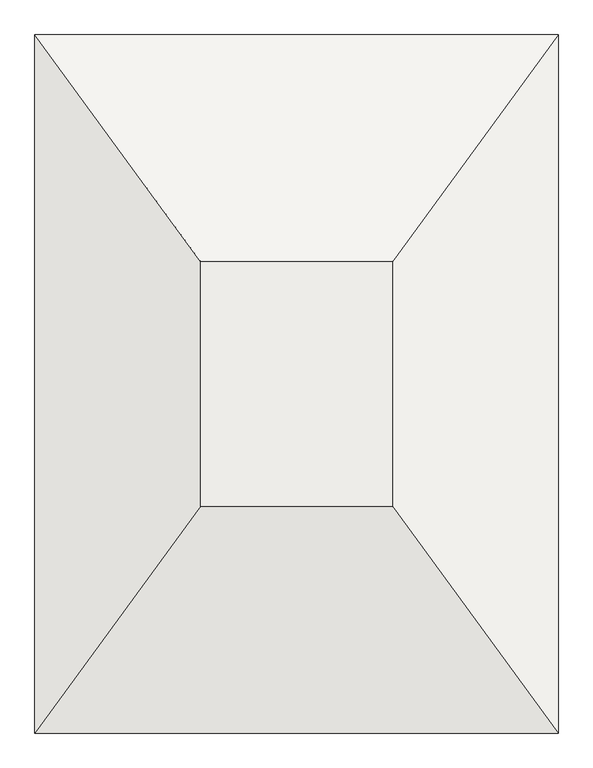
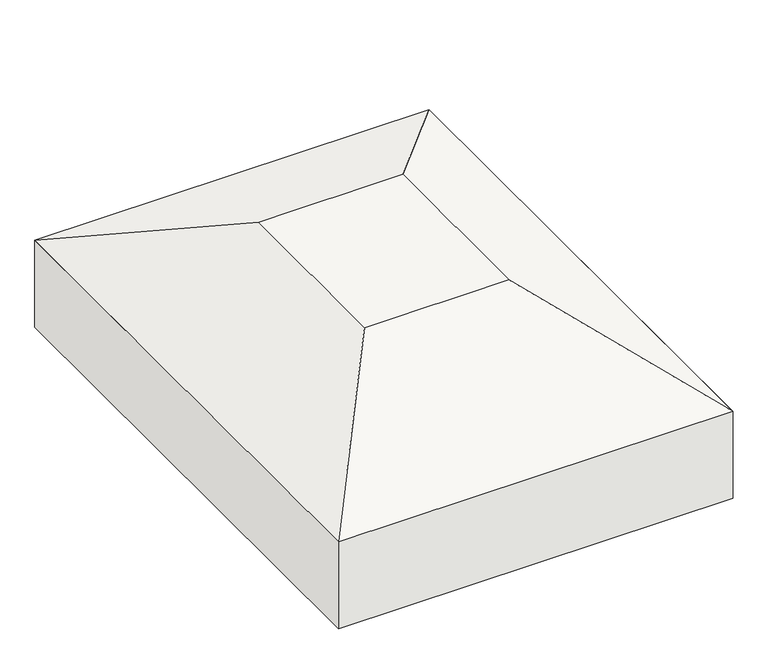
"""IFC4 building model written with IfcOpenShell, lengths in millimetres: slab geometry, 独立基础 - 坡形截面 : 独立基础 - 坡形截面."""

import ifcopenshell
import ifcopenshell.guid

model = None  # the IFC model being written
_history = None  # IfcOwnerHistory: only IFC2X3 demands one
_inside = {}  # id of a spatial element -> (the spatial element, [elements in it])
_under = {}  # id of a project, library or spatial element -> (it, [spatial elements below it])
_declared = {}  # id of a project -> (the project, [libraries it declares])
_typed = {}  # id of a type object -> (the type object, [elements of that type])
_made_of = {}  # id of a material, layer set ... -> (it, [elements and type objects made of it])


def new_model(schema):
    """Start an empty IFC model of exactly this schema.

    Asked for "IFC4X3", IfcOpenShell would pick the latest addendum, in which some entities
    have other attributes; the version numbers below select the first issue.
    IFC2X3 requires an IfcOwnerHistory on every rooted entity: one is made here for all.
    """
    global model, _history
    if schema == "IFC4X3":
        model = ifcopenshell.file(schema_version=(4, 3, 0, 0))
    else:
        model = ifcopenshell.file(schema=schema)
    _inside.clear()
    _under.clear()
    _declared.clear()
    _typed.clear()
    _made_of.clear()
    _history = None
    if model.schema == "IFC2X3":
        org = make("IfcOrganization", Name="unknown")
        user = make(
            "IfcPersonAndOrganization",
            ThePerson=make("IfcPerson", FamilyName="unknown"),
            TheOrganization=org,
        )
        app = make(
            "IfcApplication",
            ApplicationDeveloper=org,
            Version="unknown",
            ApplicationFullName="unknown",
            ApplicationIdentifier="unknown",
        )
        _history = make(
            "IfcOwnerHistory",
            OwningUser=user,
            OwningApplication=app,
            ChangeAction="ADDED",
            CreationDate=0,
        )
    return model


def make(cls, **values):
    """One entity of the class cls with the attributes given. An attribute that is None is left unset."""
    return model.create_entity(
        cls, **{name: value for name, value in values.items() if value is not None}
    )


def rooted(cls, **values):
    """An entity with a GlobalId (a new one), such as an element, a storey or a relation."""
    return make(cls, GlobalId=ifcopenshell.guid.new(), OwnerHistory=_history, **values)


def si_unit(unit_type, name, prefix=None):
    """IfcSIUnit, for example si_unit("LENGTHUNIT", "METRE", prefix="MILLI")."""
    return make("IfcSIUnit", UnitType=unit_type, Prefix=prefix, Name=name)


def assignment(units):
    """IfcUnitAssignment: the units of a project."""
    return None if units is None else make("IfcUnitAssignment", Units=units)


def point(xyz):
    """IfcCartesianPoint."""
    return None if xyz is None else make("IfcCartesianPoint", Coordinates=xyz)


def direction(xyz):
    """IfcDirection."""
    return None if xyz is None else make("IfcDirection", DirectionRatios=xyz)


def frame(location, z_axis=None, x_axis=None):
    """IfcAxis2Placement3D, a coordinate frame: its origin and axes. An axis left out is left unset."""
    return make(
        "IfcAxis2Placement3D",
        Location=point(location),
        Axis=direction(z_axis),
        RefDirection=direction(x_axis),
    )


def origin():
    """The frame at (0, 0, 0) with its axes left unset."""
    return frame((0.0, 0.0, 0.0))


def place(relative_to, where):
    """IfcLocalPlacement: puts the frame where relative to a parent placement (None: the world)."""
    return make(
        "IfcLocalPlacement", PlacementRelTo=relative_to, RelativePlacement=where
    )


def context(
    kind, dimensions, precision=None, world=None, true_north=None, identifier=None
):
    """IfcGeometricRepresentationContext, for example the 3D "Model" context."""
    return make(
        "IfcGeometricRepresentationContext",
        ContextIdentifier=identifier,
        ContextType=kind,
        CoordinateSpaceDimension=dimensions,
        Precision=precision,
        WorldCoordinateSystem=world,
        TrueNorth=true_north,
    )


def project(units=None, contexts=None):
    """IfcProject with its units and contexts."""
    return rooted(
        "IfcProject",
        Name="project",
        RepresentationContexts=contexts,
        UnitsInContext=assignment(units),
    )


def spatial(cls, under=None, at=None, **own):
    """A site, building, storey or space (cls), placed at a placement, below another one or the project."""
    s = rooted(cls, ObjectPlacement=at, **own)
    if under is not None:
        _under.setdefault(under.id(), (under, []))[1].append(s)
    return s


def polyline(points):
    """IfcPolyline through the points."""
    return make("IfcPolyline", Points=[point(p) for p in points])


def outline(outer, holes=None, kind="AREA"):
    """IfcArbitraryClosedProfileDef: a profile drawn as a closed curve; with holes, ...WithVoids."""
    if holes is None:
        return make("IfcArbitraryClosedProfileDef", ProfileType=kind, OuterCurve=outer)
    return make(
        "IfcArbitraryProfileDefWithVoids",
        ProfileType=kind,
        OuterCurve=outer,
        InnerCurves=holes,
    )


def extrude(swept, where, along, depth):
    """IfcExtrudedAreaSolid: the profile swept, set in the frame where, extruded along a direction by depth."""
    return make(
        "IfcExtrudedAreaSolid",
        SweptArea=swept,
        Position=where,
        ExtrudedDirection=direction(along),
        Depth=depth,
    )


def faces_of(points, faces, orient=None, outer=None):
    """IfcFace entities. A face is a list of loops; a loop is a list of indices into points, from 0.

    orient and outer hold one flag for each loop. By default every Orientation is true, the
    first loop of a face is its IfcFaceOuterBound and the others are IfcFaceBound.
    """
    made = []
    for i, loops in enumerate(faces):
        bounds = []
        for j, loop in enumerate(loops):
            is_outer = j == 0 if outer is None else outer[i][j]
            bounds.append(
                make(
                    "IfcFaceOuterBound" if is_outer else "IfcFaceBound",
                    Bound=make("IfcPolyLoop", Polygon=[points[k] for k in loop]),
                    Orientation=True if orient is None else orient[i][j],
                )
            )
        made.append(make("IfcFace", Bounds=bounds))
    return made


def faceted_brep(points, faces, orient=None, outer=None, voids=None):
    """IfcFacetedBrep: a solid bounded by flat faces; with voids (closed shells), ...WithVoids."""
    shared = [point(p) for p in points]
    hull = make("IfcClosedShell", CfsFaces=faces_of(shared, faces, orient, outer))
    if voids is None:
        return make("IfcFacetedBrep", Outer=hull)
    return make(
        "IfcFacetedBrepWithVoids",
        Outer=hull,
        Voids=[
            make(cls, CfsFaces=faces_of(shared, fs, o, b)) for cls, fs, o, b in voids
        ],
    )


def shape(context_of_items, identifier, shape_type, items):
    """IfcShapeRepresentation: the items that make up one representation, for example the "Body"."""
    return make(
        "IfcShapeRepresentation",
        ContextOfItems=context_of_items,
        RepresentationIdentifier=identifier,
        RepresentationType=shape_type,
        Items=items,
    )


def source(mapping_origin, context_of_items, identifier, shape_type, items):
    """IfcRepresentationMap: a shape defined once, which mapped items show again and again."""
    return make(
        "IfcRepresentationMap",
        MappingOrigin=mapping_origin,
        MappedRepresentation=shape(context_of_items, identifier, shape_type, items),
    )


def transform(
    local_origin,
    x_axis=None,
    y_axis=None,
    z_axis=None,
    scale=None,
    scale2=None,
    scale3=None,
    uniform=True,
):
    """IfcCartesianTransformationOperator3D, or its non-uniform kind. x_axis, y_axis, z_axis: its Axis1, 2, 3."""
    if uniform:
        return make(
            "IfcCartesianTransformationOperator3D",
            Axis1=direction(x_axis),
            Axis2=direction(y_axis),
            LocalOrigin=point(local_origin),
            Scale=scale,
            Axis3=direction(z_axis),
        )
    return make(
        "IfcCartesianTransformationOperator3DnonUniform",
        Axis1=direction(x_axis),
        Axis2=direction(y_axis),
        LocalOrigin=point(local_origin),
        Scale=scale,
        Axis3=direction(z_axis),
        Scale2=scale2,
        Scale3=scale3,
    )


def mapped(mapping_source, mapping_target):
    """IfcMappedItem: shows the shape of a source again, moved by a transform."""
    return make(
        "IfcMappedItem", MappingSource=mapping_source, MappingTarget=mapping_target
    )


def made_of(thing, what):
    """Note that an element or type object is made of a material, layer set ...; save() writes the relation."""
    if what is not None:
        _made_of.setdefault(what.id(), (what, []))[1].append(thing)
    return thing


def element(
    cls,
    number,
    at=None,
    inside=None,
    cuts=None,
    type_object=None,
    material=None,
    context=None,
    identifier="Body",
    shape_type=None,
    held_by="IfcProductDefinitionShape",
    body=None,
    shapes=None,
    **own,
):
    """One element of the class cls, such as IfcWall. Its Tag is "e" and its number.

    at: its placement. inside: the storey or other place that contains it. cuts: it is an
    opening in that element (IfcRelVoidsElement). A single representation is given by context,
    identifier, shape_type and body (its items); several are given by shapes. held_by: the class
    of the entity that holds the representations. save() writes the other relations.
    """
    e = rooted(cls, Tag="e%d" % number, ObjectPlacement=at, **own)
    if body is not None:
        shapes = [shape(context, identifier, shape_type, body)]
    if shapes is not None:
        e.Representation = make(held_by, Representations=shapes)
    if inside is not None:
        _inside.setdefault(inside.id(), (inside, []))[1].append(e)
    if cuts is not None:
        rooted(
            "IfcRelVoidsElement", RelatingBuildingElement=cuts, RelatedOpeningElement=e
        )
    if type_object is not None:
        _typed.setdefault(type_object.id(), (type_object, []))[1].append(e)
    return made_of(e, material)


def aggregate(whole, parts):
    """IfcRelAggregates: a whole, such as a stair, and the parts it consists of."""
    return rooted("IfcRelAggregates", RelatingObject=whole, RelatedObjects=parts)


def save(model, path):
    """Write the relations noted so far, then the file.

    IfcRelAggregates (storeys below a building ...), IfcRelContainedInSpatialStructure (elements
    in a storey), IfcRelDefinesByType, IfcRelAssociatesMaterial and IfcRelDeclares: one each for
    every whole, place, type object, material and project.
    """
    for whole, parts in _under.values():
        aggregate(whole, parts)
    for where, things in _inside.values():
        rooted(
            "IfcRelContainedInSpatialStructure",
            RelatedElements=things,
            RelatingStructure=where,
        )
    for kind, things in _typed.values():
        rooted("IfcRelDefinesByType", RelatedObjects=things, RelatingType=kind)
    for what, things in _made_of.values():
        rooted("IfcRelAssociatesMaterial", RelatedObjects=things, RelatingMaterial=what)
    for by, libraries in _declared.values():
        rooted("IfcRelDeclares", RelatingContext=by, RelatedDefinitions=libraries)
    model.write(path)


def slab_86cecf96(model_context):
    return source(origin(), model_context, "Body", "SolidModel", [
        faceted_brep([(750.0, 1000.0, -300.0), (750.0, -1000.0, -300.0), (-750.0, -1000.0, -300.0), (-750.0, 1000.0, -300.0), (275.0, 350.0, 0.0), (-275.0, 350.0, 0.0), (-275.0, -350.0, 0.0), (275.0, -350.0, 0.0)], [[[0, 1, 2, 3]], [[4, 5, 6, 7]], [[5, 4, 0, 3]], [[6, 5, 3, 2]], [[7, 6, 2, 1]], [[4, 7, 1, 0]]]),
        extrude(outline(polyline([(750.0, 1000.0), (750.0, -1000.0), (-750.0, -1000.0), (-750.0, 1000.0), (750.0, 1000.0)])), frame((0.0, 0.0, -650.0), z_axis=(0.0, 0.0, 1.0), x_axis=(1.0, 0.0, 0.0)), (0.0, 0.0, 1.0), 350.0),
    ])


if __name__ == "__main__":
    model = new_model("IFC4")
    model_context = context("Model", 3, world=origin())
    ifc_project = project(units=[si_unit("LENGTHUNIT", "METRE", prefix="MILLI")], contexts=[model_context])
    site = spatial("IfcSite", under=ifc_project)
    building = spatial("IfcBuilding", under=site)
    placement = place(None, origin())
    slab_shape = slab_86cecf96(model_context)
    element("IfcSlab", 1, ObjectType="独立基础 - 坡形截面 : 独立基础 - 坡形截面", at=placement, inside=building, context=model_context, shape_type="MappedRepresentation", body=[
        mapped(slab_shape, transform((0.0, 0.0, 0.0), x_axis=(1.0, 0.0, 0.0), y_axis=(0.0, 1.0, 0.0), z_axis=(0.0, 0.0, 1.0))),
    ])
    save(model, "model.ifc")

# Revit data of these elements
# Type "独立基础 - 坡形截面 : 独立基础 - 坡形截面"
#   h2 = 300 mm
#   h1 = 350 mm
#   d2 = 50 mm
#   d1 = 50 mm
#   Width = 1500 mm
#   Length = 2000 mm
#   Hc = 600 mm
#   Foundation Thickness = 650 mm
#   Bc = 450 mm
#   Structural Material [instance default] = 混凝土 - 现场浇注混凝土
#   Assembly Code = ""
# Element 1 (IfcSlab, "独立基础 - 坡形截面 : 独立基础 - 坡形截面")
#   Materials on its faces: "混凝土 - 现场浇注混凝土"
# Materials
#   "混凝土 - 现场浇注混凝土": class "混凝土", colour RGB 192 192 192, transparency 0
